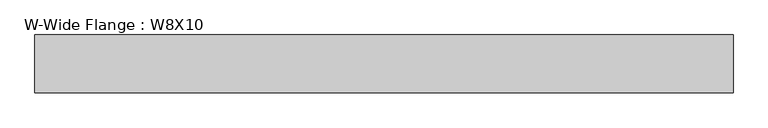
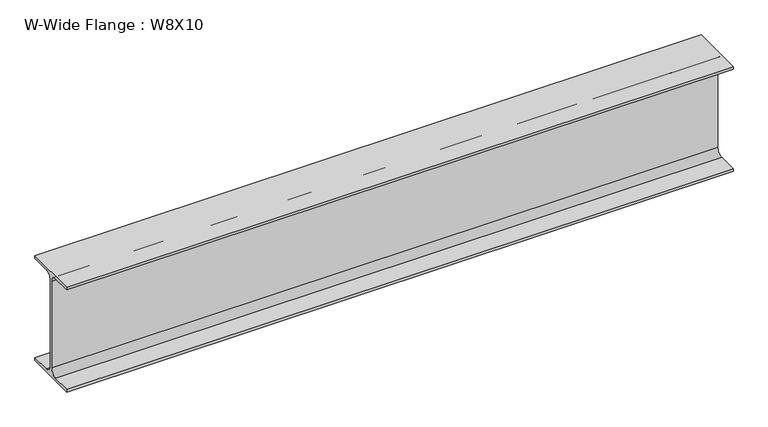
"""IFC4 building model written with IfcOpenShell, lengths in millimetres: beam geometry, W-Wide Flange : W8X10."""

from ifc_helpers import new_model, si_unit, point, frame, frame_2d, origin, place, context, project, spatial, polyline, circle_curve, trimmed, segment, composite_curve, outline, extrude, source, transform, mapped, element, save


def w_wide_flange_w8x10_8db334b5(model_context):
    return source(origin(), model_context, "Body", "SweptSolid", [
        extrude(outline(composite_curve([segment(polyline([(50.038, -94.996), (50.038, -100.203), (-50.038, -100.203), (-50.038, -94.996), (-14.4145, -94.996)]), True, "CONTINUOUS"), segment(trimmed(circle_curve(frame_2d((-14.4145, -82.7405)), 12.2555), [point((-14.4145, -94.996))], [point((-2.159, -82.7405))], True, "CARTESIAN"), True, "CONTINUOUS"), segment(polyline([(-2.159, -82.7405), (-2.159, 82.7405)]), True, "CONTINUOUS"), segment(trimmed(circle_curve(frame_2d((-14.4145, 82.7405)), 12.2555), [point((-2.159, 82.7405))], [point((-14.4145, 94.996))], True, "CARTESIAN"), True, "CONTINUOUS"), segment(polyline([(-14.4145, 94.996), (-50.038, 94.996), (-50.038, 100.203), (50.038, 100.203), (50.038, 94.996), (14.4145, 94.996)]), True, "CONTINUOUS"), segment(trimmed(circle_curve(frame_2d((14.4145, 82.7405)), 12.2555), [point((14.4145, 94.996))], [point((2.159, 82.7405))], True, "CARTESIAN"), True, "CONTINUOUS"), segment(polyline([(2.159, 82.7405), (2.159, -82.7405)]), True, "CONTINUOUS"), segment(trimmed(circle_curve(frame_2d((14.4145, -82.7405)), 12.2555), [point((2.159, -82.7405))], [point((14.4145, -94.996))], True, "CARTESIAN"), True, "CONTINUOUS"), segment(polyline([(14.4145, -94.996), (50.038, -94.996)]), True, "CONTINUOUS")], self_intersect=False)), frame((-553.767415, 0.0, 0.0), z_axis=(1.0, 0.0, 0.0), x_axis=(0.0, 1.0, 0.0)), (0.0, 0.0, 1.0), 1205.5296406),
    ])


if __name__ == "__main__":
    model = new_model("IFC4")
    model_context = context("Model", 3, world=origin())
    ifc_project = project(units=[si_unit("LENGTHUNIT", "METRE", prefix="MILLI")], contexts=[model_context])
    site = spatial("IfcSite", under=ifc_project)
    building = spatial("IfcBuilding", under=site)
    placement = place(None, origin())
    w_wide_flange_w8x10_shape = w_wide_flange_w8x10_8db334b5(model_context)
    element("IfcBeam", 1, ObjectType="W-Wide Flange : W8X10", at=placement, inside=building, context=model_context, shape_type="MappedRepresentation", body=[
        mapped(w_wide_flange_w8x10_shape, transform((0.0, 0.0, 0.0), x_axis=(1.0, 0.0, 0.0), y_axis=(0.0, 1.0, 0.0), z_axis=(0.0, 0.0, 1.0))),
    ])
    save(model, "model.ifc")

# Revit data of these elements
# Type "W-Wide Flange : W8X10"
#   Assembly Code = "B10"
#   W = 10
#   Length [instance default] = 1524 mm
#   bf = 100.076 mm
#   d = 200.406 mm
#   k = 17.463 mm
#   k2 = 12.255 mm
#   tf = 5.207 mm
#   tw = 4.318 mm
#   A = 0.00190967 m²
#   Structural Material [instance default] = Steel ASTM A992
# Element 1 (IfcBeam, "W-Wide Flange : W8X10")
#   Structural Material = Aluminum, Anodized Red
#   Materials on its faces: "Aluminum, Anodized Red"
# Materials
#   "Steel ASTM A992": class "Metal", colour RGB 128 0 0, transparency 0, Description = "Structural steel 50ksi", Cost = 0
#   "Aluminum, Anodized Red": class "Metal", colour RGB 120 120 120, transparency 0, Description = "Anodized aluminum, red", Cost = 0
